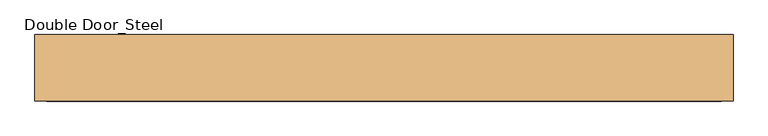
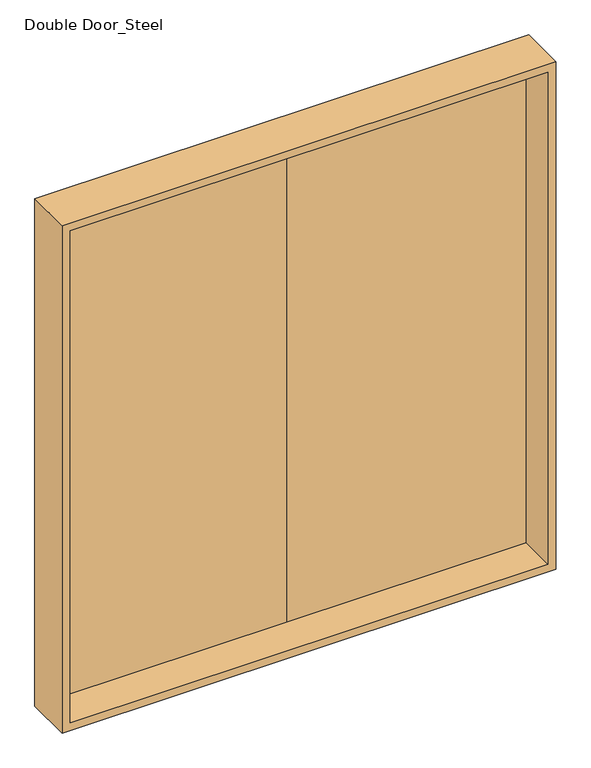
"""IFC4 building model written with IfcOpenShell, lengths in millimetres: door geometry, Double Door_Steel : H_DR_AR_B12_Double Door_Steel_W2100xH2280_FSD3."""

from ifc_helpers import new_model, si_unit, frame, origin, place, context, project, spatial, polyline, outline, extrude, faceted_brep, source, transform, mapped, element, save


def double_door_steel_a456a6a1(model_context):
    return source(origin(), model_context, "Body", "SolidModel", [
        extrude(outline(polyline([(1030.0, 60.0), (0.0, 60.0), (0.0, 100.0), (1030.0, 100.0), (1030.0, 60.0)])), frame((0.0, 0.0, 20.0), z_axis=(0.0, 0.0, 1.0), x_axis=(1.0, 0.0, 0.0)), (0.0, 0.0, 1.0), 2240.0),
        extrude(outline(polyline([(0.0, 60.0), (-1030.0, 60.0), (-1030.0, 100.0), (0.0, 100.0), (0.0, 60.0)])), frame((0.0, 0.0, 20.0), z_axis=(0.0, 0.0, 1.0), x_axis=(1.0, 0.0, 0.0)), (0.0, 0.0, 1.0), 2240.0),
        faceted_brep([(1050.0, -100.0, 2280.0), (1050.0, 100.0, 2280.0), (-1050.0, 100.0, 2280.0), (-1050.0, -100.0, 2280.0), (1015.0, 60.0, 2245.0), (1015.0, -100.0, 2245.0), (-1015.0, -100.0, 2245.0), (-1015.0, 60.0, 2245.0), (1030.0, 100.0, 2260.0), (1030.0, 60.0, 2260.0), (-1030.0, 60.0, 2260.0), (-1030.0, 100.0, 2260.0), (-1050.0, 100.0, 0.0), (-1050.0, -100.0, 0.0), (-1015.0, -100.0, 35.0), (-1015.0, 60.0, 35.0), (-1030.0, 60.0, 20.0), (-1030.0, 100.0, 20.0), (1050.0, 100.0, 0.0), (1030.0, 100.0, 20.0), (1050.0, -100.0, 0.0), (1015.0, -100.0, 35.0), (1015.0, 60.0, 35.0), (1030.0, 60.0, 20.0)], [[[0, 1, 2, 3]], [[4, 5, 6, 7]], [[8, 9, 10, 11]], [[3, 2, 12, 13]], [[7, 6, 14, 15]], [[11, 10, 16, 17]], [[18, 12, 2, 1], [8, 11, 17, 19]], [[13, 12, 18, 20]], [[0, 3, 13, 20], [21, 14, 6, 5]], [[15, 14, 21, 22]], [[23, 16, 10, 9], [4, 7, 15, 22]], [[17, 16, 23, 19]], [[20, 18, 1, 0]], [[22, 21, 5, 4]], [[19, 23, 9, 8]]]),
    ])


if __name__ == "__main__":
    model = new_model("IFC4")
    model_context = context("Model", 3, world=origin())
    ifc_project = project(units=[si_unit("LENGTHUNIT", "METRE", prefix="MILLI")], contexts=[model_context])
    site = spatial("IfcSite", under=ifc_project)
    building = spatial("IfcBuilding", under=site)
    placement = place(None, origin())
    double_door_steel_shape = double_door_steel_a456a6a1(model_context)
    element("IfcDoor", 1, ObjectType="Double Door_Steel : H_DR_AR_B12_Double Door_Steel_W2100xH2280_FSD3", at=placement, inside=building, context=model_context, shape_type="MappedRepresentation", body=[
        mapped(double_door_steel_shape, transform((0.0, 0.0, 0.0), x_axis=(1.0, 0.0, 0.0), y_axis=(0.0, 1.0, 0.0), z_axis=(0.0, 0.0, 1.0))),
    ])
    save(model, "model.ifc")

# Revit data of these elements
# Type "Double Door_Steel : H_DR_AR_B12_Double Door_Steel_W2100xH2280_FSD3"
#   Type Mark = "441"
#   프레임 = ""
#   철물 = ""
#   유리/마감 = ""
#   위치/개소 = ""
#   부호 = "1/SD"
#   문번호 = ""
#   문기호 = "SD"
#   Analytic Construction = "<None>"
#   Height = 2280 mm
#   Width = 2100 mm
#   Define Thermal Properties by = 1
#   문 틀 = none
#   문 = none
#   Function = (empty or 0)
#   Assembly Code = ""
#   Wall Closure = (empty or 0)
